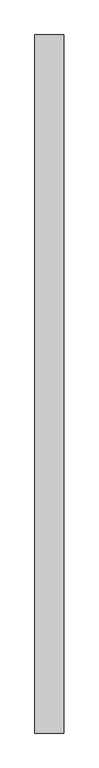
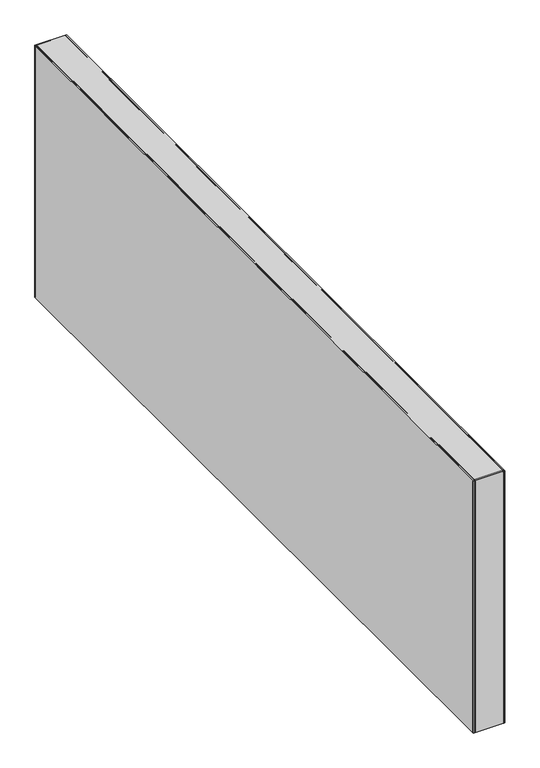
"""IFC4 building model written with IfcOpenShell, lengths in millimetres: beam geometry, LF02ZBK001_DIKE WALL_RC : Dike_Thk.250_EW3."""

from ifc_helpers import new_model, si_unit, origin, origin_with_axes, place, context, project, spatial, polyline, outline, extrude, source, transform, mapped, element, save


def beam_6e677b00(model_context):
    return source(origin(), model_context, "Body", "SweptSolid", [
        extrude(outline(polyline([(125.0, -3000.0), (-125.0, -3000.0), (-125.0, 3000.0), (125.0, 3000.0), (125.0, -3000.0)])), origin_with_axes(), (0.0, 0.0, 1.0), 2100.0),
        extrude(outline(polyline([(-125.0, -2985.0), (-125.0, -2984.0), (125.0, -2984.0), (125.0, -2985.0), (-125.0, -2985.0)])), origin_with_axes(), (0.0, 0.0, 1.0), 2100.0),
        extrude(outline(polyline([(-125.0, -2990.0), (-125.0, -2989.0), (125.0, -2989.0), (125.0, -2990.0), (-125.0, -2990.0)])), origin_with_axes(), (0.0, 0.0, 1.0), 2100.0),
        extrude(outline(polyline([(-125.0, -2995.0), (-125.0, -2994.0), (125.0, -2994.0), (125.0, -2995.0), (-125.0, -2995.0)])), origin_with_axes(), (0.0, 0.0, 1.0), 2100.0),
        extrude(outline(polyline([(-125.0, 2985.0), (125.0, 2985.0), (125.0, 2984.0), (-125.0, 2984.0), (-125.0, 2985.0)])), origin_with_axes(), (0.0, 0.0, 1.0), 2100.0),
        extrude(outline(polyline([(-125.0, 2990.0), (125.0, 2990.0), (125.0, 2989.0), (-125.0, 2989.0), (-125.0, 2990.0)])), origin_with_axes(), (0.0, 0.0, 1.0), 2100.0),
        extrude(outline(polyline([(-125.0, 2995.0), (125.0, 2995.0), (125.0, 2994.0), (-125.0, 2994.0), (-125.0, 2995.0)])), origin_with_axes(), (0.0, 0.0, 1.0), 2100.0),
        extrude(outline(polyline([(109.0, 3000.0), (110.0, 3000.0), (110.0, -3000.0), (109.0, -3000.0), (109.0, 3000.0)])), origin_with_axes(), (0.0, 0.0, 1.0), 2100.0),
        extrude(outline(polyline([(114.0, 3000.0), (115.0, 3000.0), (115.0, -3000.0), (114.0, -3000.0), (114.0, 3000.0)])), origin_with_axes(), (0.0, 0.0, 1.0), 2100.0),
        extrude(outline(polyline([(119.0, 3000.0), (120.0, 3000.0), (120.0, -3000.0), (119.0, -3000.0), (119.0, 3000.0)])), origin_with_axes(), (0.0, 0.0, 1.0), 2100.0),
        extrude(outline(polyline([(-109.0, 3000.0), (-109.0, -3000.0), (-110.0, -3000.0), (-110.0, 3000.0), (-109.0, 3000.0)])), origin_with_axes(), (0.0, 0.0, 1.0), 2100.0),
        extrude(outline(polyline([(-114.0, 3000.0), (-114.0, -3000.0), (-115.0, -3000.0), (-115.0, 3000.0), (-114.0, 3000.0)])), origin_with_axes(), (0.0, 0.0, 1.0), 2100.0),
        extrude(outline(polyline([(-119.0, 3000.0), (-119.0, -3000.0), (-120.0, -3000.0), (-120.0, 3000.0), (-119.0, 3000.0)])), origin_with_axes(), (0.0, 0.0, 1.0), 2100.0),
    ])


if __name__ == "__main__":
    model = new_model("IFC4")
    model_context = context("Model", 3, world=origin())
    ifc_project = project(units=[si_unit("LENGTHUNIT", "METRE", prefix="MILLI")], contexts=[model_context])
    site = spatial("IfcSite", under=ifc_project)
    building = spatial("IfcBuilding", under=site)
    placement = place(None, origin())
    beam_shape = beam_6e677b00(model_context)
    element("IfcBeam", 1, ObjectType="LF02ZBK001_DIKE WALL_RC : Dike_Thk.250_EW3", at=placement, inside=building, context=model_context, shape_type="MappedRepresentation", body=[
        mapped(beam_shape, transform((0.0, 0.0, 0.0), x_axis=(1.0, 0.0, 0.0), y_axis=(0.0, 1.0, 0.0), z_axis=(0.0, 0.0, 1.0))),
    ])
    save(model, "model.ifc")

# Revit data of these elements
# Type "LF02ZBK001_DIKE WALL_RC : Dike_Thk.250_EW3"
#   Dike_thk = 250 mm
#   Dike_Length [instance default] = 3000 mm
#   Dike_Hight = 2100 mm
#   c2_visible = yes
#   c3_material [instance default] = none
#   c2_material 3 [instance default] = none
#   c2_material 2 [instance default] = none
#   c2_material 1 [instance default] = none
#   c1_material [instance default] = none
#   Default Elevation = 0
# Element 1 (IfcBeam, "LF02ZBK001_DIKE WALL_RC : Dike_Thk.250_EW3")
#   Dike_Length = 6000 mm
